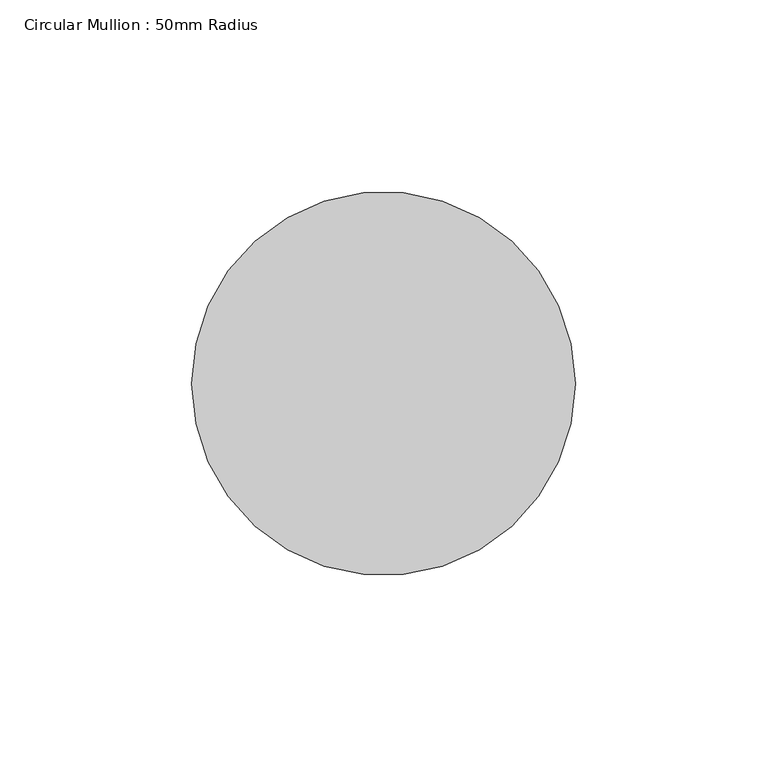
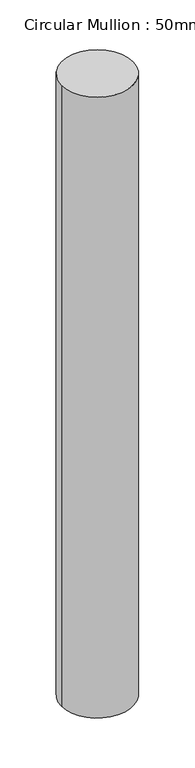
"""IFC4 building model written with IfcOpenShell, lengths in millimetres: member geometry, Circular Mullion : 50mm Radius."""

import ifcopenshell
import ifcopenshell.guid

model = None  # the IFC model being written
_history = None  # IfcOwnerHistory: only IFC2X3 demands one
_inside = {}  # id of a spatial element -> (the spatial element, [elements in it])
_under = {}  # id of a project, library or spatial element -> (it, [spatial elements below it])
_declared = {}  # id of a project -> (the project, [libraries it declares])
_typed = {}  # id of a type object -> (the type object, [elements of that type])
_made_of = {}  # id of a material, layer set ... -> (it, [elements and type objects made of it])


def new_model(schema):
    """Start an empty IFC model of exactly this schema.

    Asked for "IFC4X3", IfcOpenShell would pick the latest addendum, in which some entities
    have other attributes; the version numbers below select the first issue.
    IFC2X3 requires an IfcOwnerHistory on every rooted entity: one is made here for all.
    """
    global model, _history
    if schema == "IFC4X3":
        model = ifcopenshell.file(schema_version=(4, 3, 0, 0))
    else:
        model = ifcopenshell.file(schema=schema)
    _inside.clear()
    _under.clear()
    _declared.clear()
    _typed.clear()
    _made_of.clear()
    _history = None
    if model.schema == "IFC2X3":
        org = make("IfcOrganization", Name="unknown")
        user = make(
            "IfcPersonAndOrganization",
            ThePerson=make("IfcPerson", FamilyName="unknown"),
            TheOrganization=org,
        )
        app = make(
            "IfcApplication",
            ApplicationDeveloper=org,
            Version="unknown",
            ApplicationFullName="unknown",
            ApplicationIdentifier="unknown",
        )
        _history = make(
            "IfcOwnerHistory",
            OwningUser=user,
            OwningApplication=app,
            ChangeAction="ADDED",
            CreationDate=0,
        )
    return model


def make(cls, **values):
    """One entity of the class cls with the attributes given. An attribute that is None is left unset."""
    return model.create_entity(
        cls, **{name: value for name, value in values.items() if value is not None}
    )


def rooted(cls, **values):
    """An entity with a GlobalId (a new one), such as an element, a storey or a relation."""
    return make(cls, GlobalId=ifcopenshell.guid.new(), OwnerHistory=_history, **values)


def si_unit(unit_type, name, prefix=None):
    """IfcSIUnit, for example si_unit("LENGTHUNIT", "METRE", prefix="MILLI")."""
    return make("IfcSIUnit", UnitType=unit_type, Prefix=prefix, Name=name)


def assignment(units):
    """IfcUnitAssignment: the units of a project."""
    return None if units is None else make("IfcUnitAssignment", Units=units)


def point(xyz):
    """IfcCartesianPoint."""
    return None if xyz is None else make("IfcCartesianPoint", Coordinates=xyz)


def direction(xyz):
    """IfcDirection."""
    return None if xyz is None else make("IfcDirection", DirectionRatios=xyz)


def frame(location, z_axis=None, x_axis=None):
    """IfcAxis2Placement3D, a coordinate frame: its origin and axes. An axis left out is left unset."""
    return make(
        "IfcAxis2Placement3D",
        Location=point(location),
        Axis=direction(z_axis),
        RefDirection=direction(x_axis),
    )


def frame_2d(location, x_axis=None):
    """IfcAxis2Placement2D, a coordinate frame in the plane: its origin and x axis."""
    return make(
        "IfcAxis2Placement2D", Location=point(location), RefDirection=direction(x_axis)
    )


def origin():
    """The frame at (0, 0, 0) with its axes left unset."""
    return frame((0.0, 0.0, 0.0))


def origin_2d():
    """The frame at (0, 0) in the plane with its x axis left unset."""
    return frame_2d((0.0, 0.0))


def place(relative_to, where):
    """IfcLocalPlacement: puts the frame where relative to a parent placement (None: the world)."""
    return make(
        "IfcLocalPlacement", PlacementRelTo=relative_to, RelativePlacement=where
    )


def context(
    kind, dimensions, precision=None, world=None, true_north=None, identifier=None
):
    """IfcGeometricRepresentationContext, for example the 3D "Model" context."""
    return make(
        "IfcGeometricRepresentationContext",
        ContextIdentifier=identifier,
        ContextType=kind,
        CoordinateSpaceDimension=dimensions,
        Precision=precision,
        WorldCoordinateSystem=world,
        TrueNorth=true_north,
    )


def project(units=None, contexts=None):
    """IfcProject with its units and contexts."""
    return rooted(
        "IfcProject",
        Name="project",
        RepresentationContexts=contexts,
        UnitsInContext=assignment(units),
    )


def spatial(cls, under=None, at=None, **own):
    """A site, building, storey or space (cls), placed at a placement, below another one or the project."""
    s = rooted(cls, ObjectPlacement=at, **own)
    if under is not None:
        _under.setdefault(under.id(), (under, []))[1].append(s)
    return s


def circle_curve(where, radius):
    """IfcCircle in the frame where."""
    return make("IfcCircle", Position=where, Radius=radius)


def trimmed(basis, trim1, trim2, sense, master):
    """IfcTrimmedCurve: the piece of a basis curve between two trims."""
    return make(
        "IfcTrimmedCurve",
        BasisCurve=basis,
        Trim1=trim1,
        Trim2=trim2,
        SenseAgreement=sense,
        MasterRepresentation=master,
    )


def segment(curve, same_sense, transition):
    """IfcCompositeCurveSegment."""
    return make(
        "IfcCompositeCurveSegment",
        Transition=transition,
        SameSense=same_sense,
        ParentCurve=curve,
    )


def composite_curve(segments, self_intersect=None):
    """IfcCompositeCurve: segments joined end to end."""
    return make("IfcCompositeCurve", Segments=segments, SelfIntersect=self_intersect)


def outline(outer, holes=None, kind="AREA"):
    """IfcArbitraryClosedProfileDef: a profile drawn as a closed curve; with holes, ...WithVoids."""
    if holes is None:
        return make("IfcArbitraryClosedProfileDef", ProfileType=kind, OuterCurve=outer)
    return make(
        "IfcArbitraryProfileDefWithVoids",
        ProfileType=kind,
        OuterCurve=outer,
        InnerCurves=holes,
    )


def extrude(swept, where, along, depth):
    """IfcExtrudedAreaSolid: the profile swept, set in the frame where, extruded along a direction by depth."""
    return make(
        "IfcExtrudedAreaSolid",
        SweptArea=swept,
        Position=where,
        ExtrudedDirection=direction(along),
        Depth=depth,
    )


def shape(context_of_items, identifier, shape_type, items):
    """IfcShapeRepresentation: the items that make up one representation, for example the "Body"."""
    return make(
        "IfcShapeRepresentation",
        ContextOfItems=context_of_items,
        RepresentationIdentifier=identifier,
        RepresentationType=shape_type,
        Items=items,
    )


def source(mapping_origin, context_of_items, identifier, shape_type, items):
    """IfcRepresentationMap: a shape defined once, which mapped items show again and again."""
    return make(
        "IfcRepresentationMap",
        MappingOrigin=mapping_origin,
        MappedRepresentation=shape(context_of_items, identifier, shape_type, items),
    )


def transform(
    local_origin,
    x_axis=None,
    y_axis=None,
    z_axis=None,
    scale=None,
    scale2=None,
    scale3=None,
    uniform=True,
):
    """IfcCartesianTransformationOperator3D, or its non-uniform kind. x_axis, y_axis, z_axis: its Axis1, 2, 3."""
    if uniform:
        return make(
            "IfcCartesianTransformationOperator3D",
            Axis1=direction(x_axis),
            Axis2=direction(y_axis),
            LocalOrigin=point(local_origin),
            Scale=scale,
            Axis3=direction(z_axis),
        )
    return make(
        "IfcCartesianTransformationOperator3DnonUniform",
        Axis1=direction(x_axis),
        Axis2=direction(y_axis),
        LocalOrigin=point(local_origin),
        Scale=scale,
        Axis3=direction(z_axis),
        Scale2=scale2,
        Scale3=scale3,
    )


def mapped(mapping_source, mapping_target):
    """IfcMappedItem: shows the shape of a source again, moved by a transform."""
    return make(
        "IfcMappedItem", MappingSource=mapping_source, MappingTarget=mapping_target
    )


def made_of(thing, what):
    """Note that an element or type object is made of a material, layer set ...; save() writes the relation."""
    if what is not None:
        _made_of.setdefault(what.id(), (what, []))[1].append(thing)
    return thing


def element(
    cls,
    number,
    at=None,
    inside=None,
    cuts=None,
    type_object=None,
    material=None,
    context=None,
    identifier="Body",
    shape_type=None,
    held_by="IfcProductDefinitionShape",
    body=None,
    shapes=None,
    **own,
):
    """One element of the class cls, such as IfcWall. Its Tag is "e" and its number.

    at: its placement. inside: the storey or other place that contains it. cuts: it is an
    opening in that element (IfcRelVoidsElement). A single representation is given by context,
    identifier, shape_type and body (its items); several are given by shapes. held_by: the class
    of the entity that holds the representations. save() writes the other relations.
    """
    e = rooted(cls, Tag="e%d" % number, ObjectPlacement=at, **own)
    if body is not None:
        shapes = [shape(context, identifier, shape_type, body)]
    if shapes is not None:
        e.Representation = make(held_by, Representations=shapes)
    if inside is not None:
        _inside.setdefault(inside.id(), (inside, []))[1].append(e)
    if cuts is not None:
        rooted(
            "IfcRelVoidsElement", RelatingBuildingElement=cuts, RelatedOpeningElement=e
        )
    if type_object is not None:
        _typed.setdefault(type_object.id(), (type_object, []))[1].append(e)
    return made_of(e, material)


def aggregate(whole, parts):
    """IfcRelAggregates: a whole, such as a stair, and the parts it consists of."""
    return rooted("IfcRelAggregates", RelatingObject=whole, RelatedObjects=parts)


def save(model, path):
    """Write the relations noted so far, then the file.

    IfcRelAggregates (storeys below a building ...), IfcRelContainedInSpatialStructure (elements
    in a storey), IfcRelDefinesByType, IfcRelAssociatesMaterial and IfcRelDeclares: one each for
    every whole, place, type object, material and project.
    """
    for whole, parts in _under.values():
        aggregate(whole, parts)
    for where, things in _inside.values():
        rooted(
            "IfcRelContainedInSpatialStructure",
            RelatedElements=things,
            RelatingStructure=where,
        )
    for kind, things in _typed.values():
        rooted("IfcRelDefinesByType", RelatedObjects=things, RelatingType=kind)
    for what, things in _made_of.values():
        rooted("IfcRelAssociatesMaterial", RelatedObjects=things, RelatingMaterial=what)
    for by, libraries in _declared.values():
        rooted("IfcRelDeclares", RelatingContext=by, RelatedDefinitions=libraries)
    model.write(path)


def circular_mullion_50mm_radius_f0faa7b3(model_context):
    return source(origin(), model_context, "Body", "SweptSolid", [
        extrude(outline(composite_curve([segment(trimmed(circle_curve(origin_2d(), 50.0), [point((50.0, 0.0))], [point((-50.0, 0.0))], False, "CARTESIAN"), True, "CONTINUOUS"), segment(trimmed(circle_curve(origin_2d(), 50.0), [point((-50.0, 0.0))], [point((50.0, 0.0))], False, "CARTESIAN"), True, "CONTINUOUS")], self_intersect=False)), frame((0.0, 0.0, -919.5316848), z_axis=(0.0, 0.0, 1.0), x_axis=(1.0, 0.0, 0.0)), (0.0, 0.0, 1.0), 919.5316848),
    ])


if __name__ == "__main__":
    model = new_model("IFC4")
    model_context = context("Model", 3, world=origin())
    ifc_project = project(units=[si_unit("LENGTHUNIT", "METRE", prefix="MILLI")], contexts=[model_context])
    site = spatial("IfcSite", under=ifc_project)
    building = spatial("IfcBuilding", under=site)
    placement = place(None, origin())
    circular_mullion_50mm_radius_shape = circular_mullion_50mm_radius_f0faa7b3(model_context)
    element("IfcMember", 1, ObjectType="Circular Mullion : 50mm Radius", at=placement, inside=building, context=model_context, shape_type="MappedRepresentation", body=[
        mapped(circular_mullion_50mm_radius_shape, transform((0.0, 0.0, 0.0), x_axis=(1.0, 0.0, 0.0), y_axis=(0.0, 1.0, 0.0), z_axis=(0.0, 0.0, 1.0))),
    ])
    save(model, "model.ifc")

# Revit data of these elements
# Type "Circular Mullion : 50mm Radius"
#   built-in parameter 1007350 = 0.164042 (stored number, unit not read)
# Element 1 (IfcMember, "Circular Mullion : 50mm Radius")
#   Materials on its faces: "Aluminium"
# Materials
#   "Aluminium": class "Metal", colour RGB 247 247 247, transparency 0, Description = "Aluminium 6061", Cost = 0
